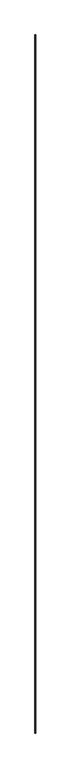
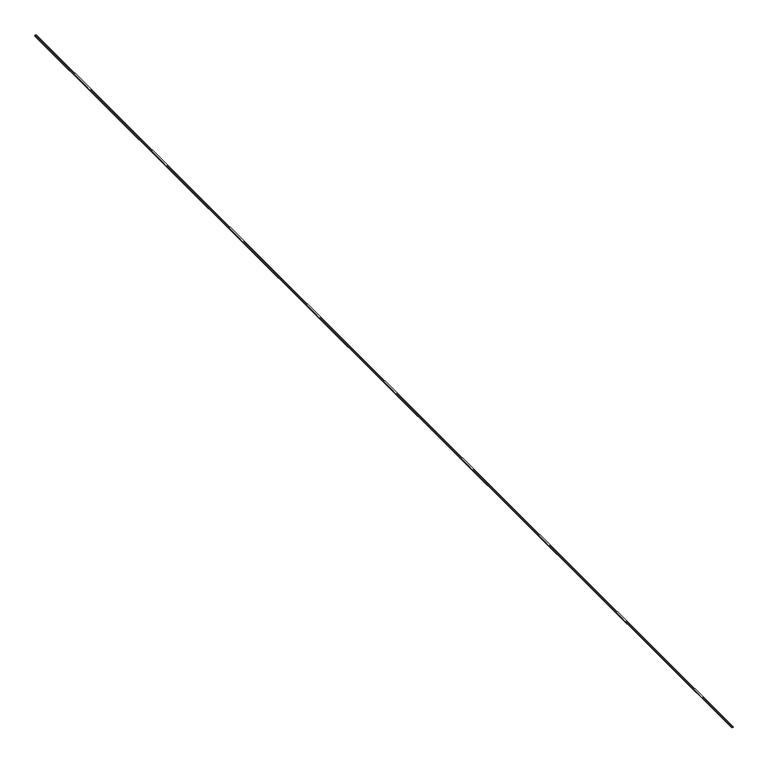
"""IFC4 building model written with IfcOpenShell, lengths in millimetres: proxy geometry, Generic Models 3:Generic Models 1:4:Generic Models 1:4 : Generic Models 3:Generic Models 1:300625:1:Generic Models 1:4:Generic Models 1:4 : Generic Models 3:Generic Models 1:300625:1 : Generic Models 3:Generic Models 1:4:Generic Models 1:4 : Generic Models 3:Generic Models 1:300625:338780:1 : Generic Models 3:Generic Models 1:4:Generic Models 1:4 : Generic Models 3:Generic Models 1:300625:1:Generic Models 1:4:Generic Models 1:4 : Generic Models 3:Generic Models 1:300625:1 : Generic Models 3:Generic Models 1:4:Generic Models 1:4 : Generic Models 3:Generic Models 1:300625:338780:317135."""

from ifc_helpers import new_model, si_unit, frame, origin, place, context, project, spatial, polyline, outline, extrude, source, transform, mapped, element, save


def generic_models_b6f82bf1(model_context):
    return source(origin(), model_context, "Body", "SweptSolid", [
        extrude(outline(polyline([(3713.8232545, 560277.8791785), (3714.4746585, 560277.3325857), (3715.4107545, 560277.0817595), (3716.3468505, 560277.3325857), (3716.9982545, 560277.8791785), (3716.9982545, 560271.6918357), (3716.3468505, 560272.2384285), (3715.4107545, 560272.4892547), (3714.4746585, 560272.2384285), (3713.8232545, 560271.6918357), (3713.8232545, 560277.8791785)])), frame((0.0, -548060.3163841, 0.0), z_axis=(0.0, 1.0, 0.0), x_axis=(0.0, 0.0, 1.0)), (0.0, 0.0, 1.0), 4876.8),
    ])


if __name__ == "__main__":
    model = new_model("IFC4")
    model_context = context("Model", 3, world=origin())
    ifc_project = project(units=[si_unit("LENGTHUNIT", "METRE", prefix="MILLI")], contexts=[model_context])
    site = spatial("IfcSite", under=ifc_project)
    building = spatial("IfcBuilding", under=site)
    placement = place(None, origin())
    generic_models_shape = generic_models_b6f82bf1(model_context)
    element("IfcBuildingElementProxy", 1, Name="Generic Models 3:Generic Models 1:4:Generic Models 1:4 : Generic Models 3:Generic Models 1:300625:1:Generic Models 1:4:Generic Models 1:4 : Generic Models 3:Generic Models 1:300625:1 : Generic Models 3:Generic Models 1:4:Generic Models 1:4 : Generic Models 3:Generic Models 1:300625:338780:1 : Generic Models 3:Generic Models 1:4:Generic Models 1:4 : Generic Models 3:Generic Models 1:300625:1:Generic Models 1:4:Generic Models 1:4 : Generic Models 3:Generic Models 1:300625:1 : Generic Models 3:Generic Models 1:4:Generic Models 1:4 : Generic Models 3:Generic Models 1:300625:338780:317135", ObjectType="Generic Models 3:Generic Models 1:4:Generic Models 1:4 : Generic Models 3:Generic Models 1:300625:1:Generic Models 1:4:Generic Models 1:4 : Generic Models 3:Generic Models 1:300625:1 : Generic Models 3:Generic Models 1:4:Generic Models 1:4 : Generic Models 3:Generic Models 1:300625:338780:1 : Generic Models 3:Generic Models 1:4:Generic Models 1:4 : Generic Models 3:Generic Models 1:300625:1:Generic Models 1:4:Generic Models 1:4 : Generic Models 3:Generic Models 1:300625:1 : Generic Models 3:Generic Models 1:4:Generic Models 1:4 : Generic Models 3:Generic Models 1:300625:338780:317135", at=placement, inside=building, context=model_context, shape_type="MappedRepresentation", body=[
        mapped(generic_models_shape, transform((0.0, 0.0, 0.0), x_axis=(1.0, 0.0, 0.0), y_axis=(0.0, 1.0, 0.0), z_axis=(0.0, 0.0, 1.0))),
    ])
    save(model, "model.ifc")

# Revit data of these elements
# Type "Generic Models 3:Generic Models 1:4:Generic Models 1:4 : Generic Models 3:Generic Models 1:300625:1:Generic Models 1:4:Generic Models 1:4 : Generic Models 3:Generic Models 1:300625:1 : Generic Models 3:Generic Models 1:4:Generic Models 1:4 : Generic Models 3:Generic Models 1:300625:338780:1 : Generic Models 3:Generic Models 1:4:Generic Models 1:4 : Generic Models 3:Generic Models 1:300625:1:Generic Models 1:4:Generic Models 1:4 : Generic Models 3:Generic Models 1:300625:1 : Generic Models 3:Generic Models 1:4:Generic Models 1:4 : Generic Models 3:Generic Models 1:300625:338780:317135"
#   NameOverride = "Generic Models 3:Generic Models 1:4:Generic Models 1:4 : Generic Models 3:Generic Models 1:300625:1:Generic Models 1:4:Generic Models 1:4 : Generic Models 3:Generic Models 1:300625:1 : Generic Models 3:Generic Models 1:4:Generic Models 1:4 : Generic Models 3:Generic Models 1:300625:338780:317135"
#   ObjectTypeOverride = "Generic Models 1:4:Generic Models 1:4 : Generic Models 3:Generic Models 1:300625:1 : Generic Models 3:Generic Models 1:4:Generic Models 1:4 : Generic Models 3:Generic Models 1:300625:338780"
#   Reference = "Generic Models 1"
#   Tag = "317135"
# Element 1 (IfcBuildingElementProxy, "Generic Models 3:Generic Models 1:4:Generic Models 1:4 : Generic Models 3:Generic Models 1:300625:1:Generic Models 1:4:Generic Models 1:4 : Generic Models 3:Generic Models 1:300625:1 : Generic Models 3:Generic Models 1:4:Generic Models 1:4 : Generic Models 3:Generic Models 1:300625:338780:1 : Generic Models 3:Generic Models 1:4:Generic Models 1:4 : Generic Models 3:Generic Models 1:300625:1:Generic Models 1:4:Generic Models 1:4 : Generic Models 3:Generic Models 1:300625:1 : Generic Models 3:Generic Models 1:4:Generic Models 1:4 : Generic Models 3:Generic Models 1:300625:338780:317135")
#   Materials on its faces: "SEALANT & BACKER ROD, IF NECESSARY"
# Materials
#   "SEALANT & BACKER ROD, IF NECESSARY": class "Unassigned", colour RGB 120 120 120, transparency 0, Cost = 0
